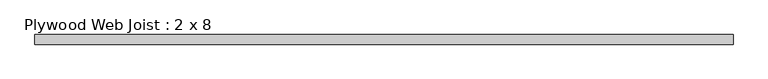
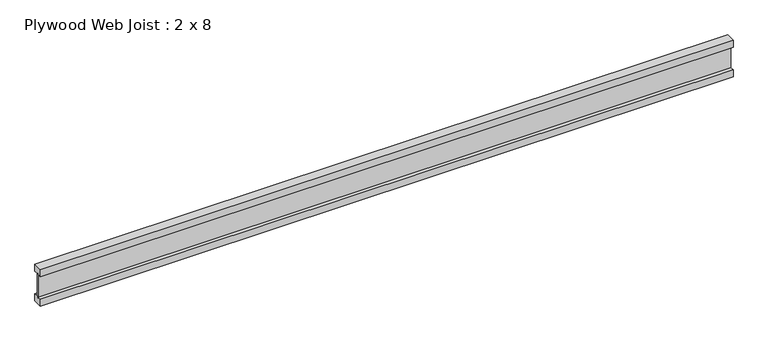
"""IFC4 building model written with IfcOpenShell, lengths in millimetres: beam geometry, Plywood Web Joist : 2 x 8."""

from ifc_helpers import new_model, si_unit, frame, origin, place, context, project, spatial, polyline, outline, extrude, source, transform, mapped, element, save


def plywood_web_joist_2_x_8_093a3c26(model_context):
    return source(origin(), model_context, "Body", "SweptSolid", [
        extrude(outline(polyline([(-25.4, 101.6), (25.4, 101.6), (25.4, 63.5), (4.7625, 63.5), (4.7625, 69.85), (-4.7625, 69.85), (-4.7625, 63.5), (-25.4, 63.5), (-25.4, 101.6)])), frame((-1835.15, 0.0, 0.0), z_axis=(1.0, 0.0, 0.0), x_axis=(0.0, 1.0, 0.0)), (0.0, 0.0, 1.0), 3670.3),
        extrude(outline(polyline([(25.4, -63.5), (25.4, -101.6), (-25.4, -101.6), (-25.4, -63.5), (-4.7625, -63.5), (-4.7625, -69.1160374), (4.7625, -69.1160374), (4.7625, -63.5), (25.4, -63.5)])), frame((-1835.15, 0.0, 0.0), z_axis=(1.0, 0.0, 0.0), x_axis=(0.0, 1.0, 0.0)), (0.0, 0.0, 1.0), 3670.3),
        extrude(outline(polyline([(1835.15, 4.7625), (1835.15, -4.7625), (-1835.15, -4.7625), (-1835.15, 4.7625), (1835.15, 4.7625)])), frame((0.0, 0.0, -69.1160374), z_axis=(0.0, 0.0, 1.0), x_axis=(1.0, 0.0, 0.0)), (0.0, 0.0, 1.0), 138.9660374),
    ])


if __name__ == "__main__":
    model = new_model("IFC4")
    model_context = context("Model", 3, world=origin())
    ifc_project = project(units=[si_unit("LENGTHUNIT", "METRE", prefix="MILLI")], contexts=[model_context])
    site = spatial("IfcSite", under=ifc_project)
    building = spatial("IfcBuilding", under=site)
    placement = place(None, origin())
    plywood_web_joist_2_x_8_shape = plywood_web_joist_2_x_8_093a3c26(model_context)
    element("IfcBeam", 1, ObjectType="Plywood Web Joist : 2 x 8", at=placement, inside=building, context=model_context, shape_type="MappedRepresentation", body=[
        mapped(plywood_web_joist_2_x_8_shape, transform((0.0, 0.0, 0.0), x_axis=(1.0, 0.0, 0.0), y_axis=(0.0, 1.0, 0.0), z_axis=(0.0, 0.0, 1.0))),
    ])
    save(model, "model.ifc")

# Revit data of these elements
# Type "Plywood Web Joist : 2 x 8"
#   Assembly Code = "B10"
#   Length [instance default] = 5' - 0"
#   b = 0' - 2"
#   d = 0' - 8"
#   Structural Material [instance default] = Softwood, Lumber
# Element 1 (IfcBeam, "Plywood Web Joist : 2 x 8")
#   Materials on its faces: "Softwood, Lumber"
# Materials
#   "Softwood, Lumber": class "Wood", colour RGB 144 113 62, transparency 0, Description = "Pinus Echinata", Cost = 0
